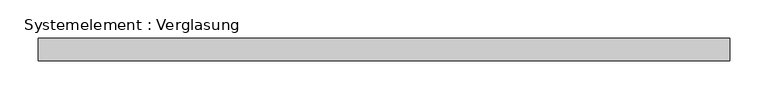
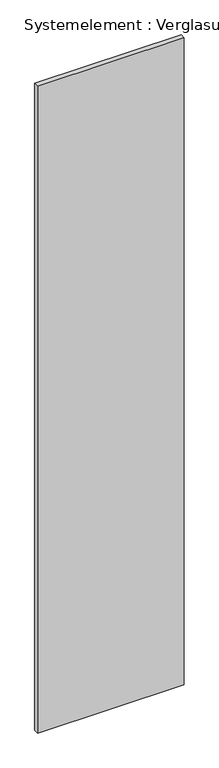
"""IFC4 building model written with IfcOpenShell, lengths in millimetres: plate geometry, Systemelement : Verglasung."""

from ifc_helpers import new_model, si_unit, origin, origin_with_axes, place, context, project, spatial, polyline, outline, extrude, source, transform, mapped, element, save


def systemelement_verglasung_88631e7e(model_context):
    return source(origin(), model_context, "Body", "SweptSolid", [
        extrude(outline(polyline([(454.4820562, -15.0), (-454.4820562, -15.0), (-454.4820562, 15.0), (454.4820562, 15.0), (454.4820562, -15.0)])), origin_with_axes(), (0.0, 0.0, 1.0), 4236.6788019),
    ])


if __name__ == "__main__":
    model = new_model("IFC4")
    model_context = context("Model", 3, world=origin())
    ifc_project = project(units=[si_unit("LENGTHUNIT", "METRE", prefix="MILLI")], contexts=[model_context])
    site = spatial("IfcSite", under=ifc_project)
    building = spatial("IfcBuilding", under=site)
    placement = place(None, origin())
    systemelement_verglasung_shape = systemelement_verglasung_88631e7e(model_context)
    element("IfcPlate", 1, ObjectType="Systemelement : Verglasung", at=placement, inside=building, context=model_context, shape_type="MappedRepresentation", body=[
        mapped(systemelement_verglasung_shape, transform((0.0, 0.0, 0.0), x_axis=(1.0, 0.0, 0.0), y_axis=(0.0, 1.0, 0.0), z_axis=(0.0, 0.0, 1.0))),
    ])
    save(model, "model.ifc")

# Revit data of these elements
# Type "Systemelement : Verglasung"
#   Construction Type Id = "GSP4R"
#   Analytic Construction = "1/8 Zoll Pilkington-Verglasung einfach"
#   Visual Light Transmittance = 0.9
#   Solar Heat Gain Coefficient = 0.86
#   Heat Transfer Coefficient (U) = 6.7069 W/(m²·K)
# Element 1 (IfcPlate, "Systemelement : Verglasung")
#   Materials on its faces: "Glas"
# Materials
#   "Glas": class "Glas", colour RGB 0 0 255, transparency 0.75, Comments = "Render-Darstellung nicht aktualisiert ", Cost = 0
